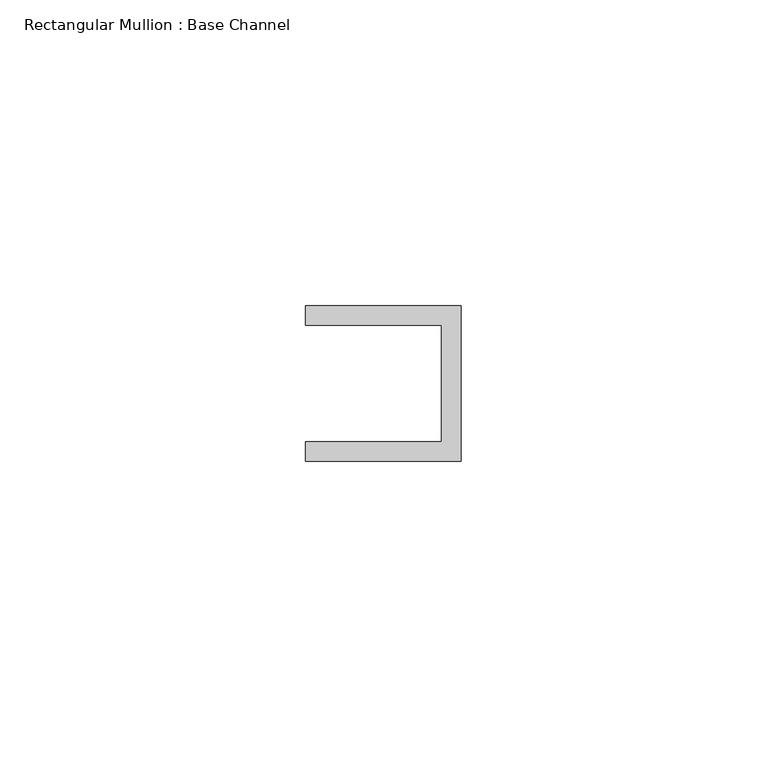
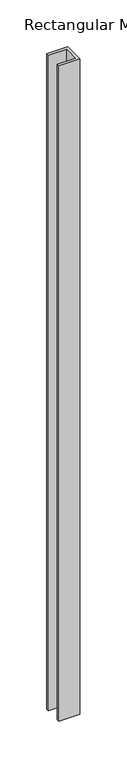
"""IFC4 building model written with IfcOpenShell, lengths in millimetres: member geometry, Rectangular Mullion : Base Channel."""

import ifcopenshell
import ifcopenshell.guid

model = None  # the IFC model being written
_history = None  # IfcOwnerHistory: only IFC2X3 demands one
_inside = {}  # id of a spatial element -> (the spatial element, [elements in it])
_under = {}  # id of a project, library or spatial element -> (it, [spatial elements below it])
_declared = {}  # id of a project -> (the project, [libraries it declares])
_typed = {}  # id of a type object -> (the type object, [elements of that type])
_made_of = {}  # id of a material, layer set ... -> (it, [elements and type objects made of it])


def new_model(schema):
    """Start an empty IFC model of exactly this schema.

    Asked for "IFC4X3", IfcOpenShell would pick the latest addendum, in which some entities
    have other attributes; the version numbers below select the first issue.
    IFC2X3 requires an IfcOwnerHistory on every rooted entity: one is made here for all.
    """
    global model, _history
    if schema == "IFC4X3":
        model = ifcopenshell.file(schema_version=(4, 3, 0, 0))
    else:
        model = ifcopenshell.file(schema=schema)
    _inside.clear()
    _under.clear()
    _declared.clear()
    _typed.clear()
    _made_of.clear()
    _history = None
    if model.schema == "IFC2X3":
        org = make("IfcOrganization", Name="unknown")
        user = make(
            "IfcPersonAndOrganization",
            ThePerson=make("IfcPerson", FamilyName="unknown"),
            TheOrganization=org,
        )
        app = make(
            "IfcApplication",
            ApplicationDeveloper=org,
            Version="unknown",
            ApplicationFullName="unknown",
            ApplicationIdentifier="unknown",
        )
        _history = make(
            "IfcOwnerHistory",
            OwningUser=user,
            OwningApplication=app,
            ChangeAction="ADDED",
            CreationDate=0,
        )
    return model


def make(cls, **values):
    """One entity of the class cls with the attributes given. An attribute that is None is left unset."""
    return model.create_entity(
        cls, **{name: value for name, value in values.items() if value is not None}
    )


def rooted(cls, **values):
    """An entity with a GlobalId (a new one), such as an element, a storey or a relation."""
    return make(cls, GlobalId=ifcopenshell.guid.new(), OwnerHistory=_history, **values)


def si_unit(unit_type, name, prefix=None):
    """IfcSIUnit, for example si_unit("LENGTHUNIT", "METRE", prefix="MILLI")."""
    return make("IfcSIUnit", UnitType=unit_type, Prefix=prefix, Name=name)


def assignment(units):
    """IfcUnitAssignment: the units of a project."""
    return None if units is None else make("IfcUnitAssignment", Units=units)


def point(xyz):
    """IfcCartesianPoint."""
    return None if xyz is None else make("IfcCartesianPoint", Coordinates=xyz)


def direction(xyz):
    """IfcDirection."""
    return None if xyz is None else make("IfcDirection", DirectionRatios=xyz)


def frame(location, z_axis=None, x_axis=None):
    """IfcAxis2Placement3D, a coordinate frame: its origin and axes. An axis left out is left unset."""
    return make(
        "IfcAxis2Placement3D",
        Location=point(location),
        Axis=direction(z_axis),
        RefDirection=direction(x_axis),
    )


def origin():
    """The frame at (0, 0, 0) with its axes left unset."""
    return frame((0.0, 0.0, 0.0))


def place(relative_to, where):
    """IfcLocalPlacement: puts the frame where relative to a parent placement (None: the world)."""
    return make(
        "IfcLocalPlacement", PlacementRelTo=relative_to, RelativePlacement=where
    )


def context(
    kind, dimensions, precision=None, world=None, true_north=None, identifier=None
):
    """IfcGeometricRepresentationContext, for example the 3D "Model" context."""
    return make(
        "IfcGeometricRepresentationContext",
        ContextIdentifier=identifier,
        ContextType=kind,
        CoordinateSpaceDimension=dimensions,
        Precision=precision,
        WorldCoordinateSystem=world,
        TrueNorth=true_north,
    )


def project(units=None, contexts=None):
    """IfcProject with its units and contexts."""
    return rooted(
        "IfcProject",
        Name="project",
        RepresentationContexts=contexts,
        UnitsInContext=assignment(units),
    )


def spatial(cls, under=None, at=None, **own):
    """A site, building, storey or space (cls), placed at a placement, below another one or the project."""
    s = rooted(cls, ObjectPlacement=at, **own)
    if under is not None:
        _under.setdefault(under.id(), (under, []))[1].append(s)
    return s


def polyline(points):
    """IfcPolyline through the points."""
    return make("IfcPolyline", Points=[point(p) for p in points])


def outline(outer, holes=None, kind="AREA"):
    """IfcArbitraryClosedProfileDef: a profile drawn as a closed curve; with holes, ...WithVoids."""
    if holes is None:
        return make("IfcArbitraryClosedProfileDef", ProfileType=kind, OuterCurve=outer)
    return make(
        "IfcArbitraryProfileDefWithVoids",
        ProfileType=kind,
        OuterCurve=outer,
        InnerCurves=holes,
    )


def extrude(swept, where, along, depth):
    """IfcExtrudedAreaSolid: the profile swept, set in the frame where, extruded along a direction by depth."""
    return make(
        "IfcExtrudedAreaSolid",
        SweptArea=swept,
        Position=where,
        ExtrudedDirection=direction(along),
        Depth=depth,
    )


def shape(context_of_items, identifier, shape_type, items):
    """IfcShapeRepresentation: the items that make up one representation, for example the "Body"."""
    return make(
        "IfcShapeRepresentation",
        ContextOfItems=context_of_items,
        RepresentationIdentifier=identifier,
        RepresentationType=shape_type,
        Items=items,
    )


def source(mapping_origin, context_of_items, identifier, shape_type, items):
    """IfcRepresentationMap: a shape defined once, which mapped items show again and again."""
    return make(
        "IfcRepresentationMap",
        MappingOrigin=mapping_origin,
        MappedRepresentation=shape(context_of_items, identifier, shape_type, items),
    )


def transform(
    local_origin,
    x_axis=None,
    y_axis=None,
    z_axis=None,
    scale=None,
    scale2=None,
    scale3=None,
    uniform=True,
):
    """IfcCartesianTransformationOperator3D, or its non-uniform kind. x_axis, y_axis, z_axis: its Axis1, 2, 3."""
    if uniform:
        return make(
            "IfcCartesianTransformationOperator3D",
            Axis1=direction(x_axis),
            Axis2=direction(y_axis),
            LocalOrigin=point(local_origin),
            Scale=scale,
            Axis3=direction(z_axis),
        )
    return make(
        "IfcCartesianTransformationOperator3DnonUniform",
        Axis1=direction(x_axis),
        Axis2=direction(y_axis),
        LocalOrigin=point(local_origin),
        Scale=scale,
        Axis3=direction(z_axis),
        Scale2=scale2,
        Scale3=scale3,
    )


def mapped(mapping_source, mapping_target):
    """IfcMappedItem: shows the shape of a source again, moved by a transform."""
    return make(
        "IfcMappedItem", MappingSource=mapping_source, MappingTarget=mapping_target
    )


def made_of(thing, what):
    """Note that an element or type object is made of a material, layer set ...; save() writes the relation."""
    if what is not None:
        _made_of.setdefault(what.id(), (what, []))[1].append(thing)
    return thing


def element(
    cls,
    number,
    at=None,
    inside=None,
    cuts=None,
    type_object=None,
    material=None,
    context=None,
    identifier="Body",
    shape_type=None,
    held_by="IfcProductDefinitionShape",
    body=None,
    shapes=None,
    **own,
):
    """One element of the class cls, such as IfcWall. Its Tag is "e" and its number.

    at: its placement. inside: the storey or other place that contains it. cuts: it is an
    opening in that element (IfcRelVoidsElement). A single representation is given by context,
    identifier, shape_type and body (its items); several are given by shapes. held_by: the class
    of the entity that holds the representations. save() writes the other relations.
    """
    e = rooted(cls, Tag="e%d" % number, ObjectPlacement=at, **own)
    if body is not None:
        shapes = [shape(context, identifier, shape_type, body)]
    if shapes is not None:
        e.Representation = make(held_by, Representations=shapes)
    if inside is not None:
        _inside.setdefault(inside.id(), (inside, []))[1].append(e)
    if cuts is not None:
        rooted(
            "IfcRelVoidsElement", RelatingBuildingElement=cuts, RelatedOpeningElement=e
        )
    if type_object is not None:
        _typed.setdefault(type_object.id(), (type_object, []))[1].append(e)
    return made_of(e, material)


def aggregate(whole, parts):
    """IfcRelAggregates: a whole, such as a stair, and the parts it consists of."""
    return rooted("IfcRelAggregates", RelatingObject=whole, RelatedObjects=parts)


def save(model, path):
    """Write the relations noted so far, then the file.

    IfcRelAggregates (storeys below a building ...), IfcRelContainedInSpatialStructure (elements
    in a storey), IfcRelDefinesByType, IfcRelAssociatesMaterial and IfcRelDeclares: one each for
    every whole, place, type object, material and project.
    """
    for whole, parts in _under.values():
        aggregate(whole, parts)
    for where, things in _inside.values():
        rooted(
            "IfcRelContainedInSpatialStructure",
            RelatedElements=things,
            RelatingStructure=where,
        )
    for kind, things in _typed.values():
        rooted("IfcRelDefinesByType", RelatedObjects=things, RelatingType=kind)
    for what, things in _made_of.values():
        rooted("IfcRelAssociatesMaterial", RelatedObjects=things, RelatingMaterial=what)
    for by, libraries in _declared.values():
        rooted("IfcRelDeclares", RelatingContext=by, RelatedDefinitions=libraries)
    model.write(path)


def rectangular_mullion_base_channel_ea7c2e90(model_context):
    return source(origin(), model_context, "Body", "SweptSolid", [
        extrude(outline(polyline([(0.0, -12.7), (-25.4, -12.7), (-25.4, -9.525), (-3.175, -9.525), (-3.175, 9.525), (-25.4, 9.525), (-25.4, 12.7), (0.0, 12.7), (0.0, -12.7)])), frame((0.0, 0.0, -851.126786), z_axis=(0.0, 0.0, 1.0), x_axis=(1.0, 0.0, 0.0)), (0.0, 0.0, 1.0), 851.126786),
    ])


if __name__ == "__main__":
    model = new_model("IFC4")
    model_context = context("Model", 3, world=origin())
    ifc_project = project(units=[si_unit("LENGTHUNIT", "METRE", prefix="MILLI")], contexts=[model_context])
    site = spatial("IfcSite", under=ifc_project)
    building = spatial("IfcBuilding", under=site)
    placement = place(None, origin())
    rectangular_mullion_base_channel_shape = rectangular_mullion_base_channel_ea7c2e90(model_context)
    element("IfcMember", 1, ObjectType="Rectangular Mullion : Base Channel", at=placement, inside=building, context=model_context, shape_type="MappedRepresentation", body=[
        mapped(rectangular_mullion_base_channel_shape, transform((0.0, 0.0, 0.0), x_axis=(1.0, 0.0, 0.0), y_axis=(0.0, 1.0, 0.0), z_axis=(0.0, 0.0, 1.0))),
    ])
    save(model, "model.ifc")

# Revit data of these elements
# Type "Rectangular Mullion : Base Channel"
#   built-in parameter 1007322 = 0.0833333 (stored number, unit not read)
#   built-in parameter 1007321 = 0.0416667 (stored number, unit not read)
#   built-in parameter 1007320 = -0.03125 (stored number, unit not read)
# Element 1 (IfcMember, "Rectangular Mullion : Base Channel")
#   Materials on its faces: "ALUM"
# Materials
#   "ALUM": class "Generic", colour RGB 157 157 157, transparency 0, Cost = 0
